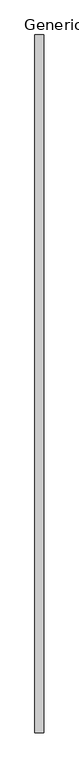
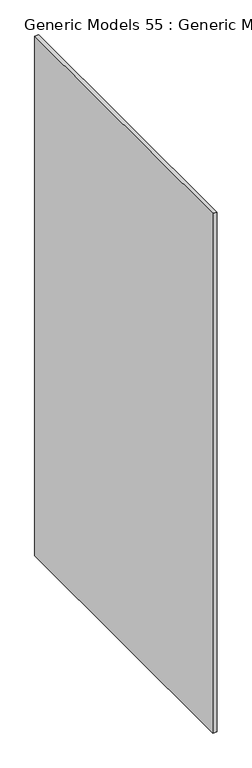
"""IFC4 building model written with IfcOpenShell, lengths in millimetres: proxy geometry, Generic Models 55 : Generic Models 1."""

from ifc_helpers import new_model, si_unit, frame, origin, place, context, project, spatial, polyline, outline, extrude, source, transform, mapped, element, save


def generic_models_55_generic_models_1_42571d6e(model_context):
    return source(origin(), model_context, "Body", "SweptSolid", [
        extrude(outline(polyline([(52238.275, 1219.2), (52238.275, 0.0), (52222.4, 0.0), (52222.4, 1219.2), (52238.275, 1219.2)])), frame((0.0, 0.0, 3054.35), z_axis=(0.0, 0.0, 1.0), x_axis=(1.0, 0.0, 0.0)), (0.0, 0.0, 1.0), 2168.128125),
    ])


if __name__ == "__main__":
    model = new_model("IFC4")
    model_context = context("Model", 3, world=origin())
    ifc_project = project(units=[si_unit("LENGTHUNIT", "METRE", prefix="MILLI")], contexts=[model_context])
    site = spatial("IfcSite", under=ifc_project)
    building = spatial("IfcBuilding", under=site)
    placement = place(None, origin())
    generic_models_55_generic_models_1_shape = generic_models_55_generic_models_1_42571d6e(model_context)
    element("IfcBuildingElementProxy", 1, Name="Generic Models 55 : Generic Models 1", ObjectType="Generic Models 55 : Generic Models 1", at=placement, inside=building, context=model_context, shape_type="MappedRepresentation", body=[
        mapped(generic_models_55_generic_models_1_shape, transform((0.0, 0.0, 0.0), x_axis=(1.0, 0.0, 0.0), y_axis=(0.0, 1.0, 0.0), z_axis=(0.0, 0.0, 1.0))),
    ])
    save(model, "model.ifc")

# Revit data of these elements
# Element 1 (IfcBuildingElementProxy, "Generic Models 55 : Generic Models 1")
#   Materials on its faces: "5/8\" GYP. BD"
# Materials
#   "5/8\" GYP. BD": class "Generic", colour RGB 255 255 255, transparency 0, Description = "Gypsum Wall Board", Cost = 0
